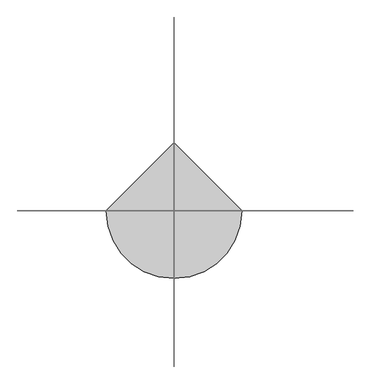
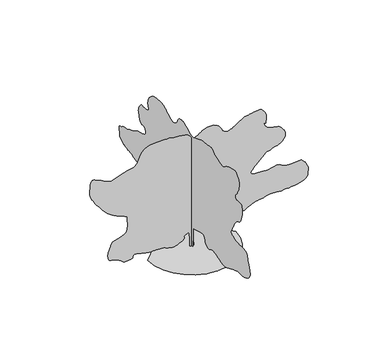
"""IFC4 building model written with IfcOpenShell, lengths in millimetres: geographic element geometry, RPC 木 - 落葉樹 : ヤマボウシ - 3.0 メートル."""

from ifc_helpers import new_model, si_unit, origin, place, context, project, spatial, triangles, source, transform, mapped, element, save


def geographic_element_e0625334(model_context):
    return source(origin(), model_context, "Body", "Tessellation", [
        triangles([(0.0321152, 48.5607305, 0.0034119), (0.0321152, -50.059231, 0.0034119), (0.0321152, -56.2224767, 326.6823853), (0.0321152, -56.2224767, 468.4473149), (0.0321152, -179.4974194, 505.4297959), (0.0321152, -382.8998477, 573.2297636), (0.0321152, -481.5198092, 585.5572815), (0.0321152, -493.3798047, 574.9372539), (0.0321152, -505.079781, 563.9947895), (0.0321152, -516.4547771, 552.4022922), (0.0321152, -527.3447737, 539.8422667), (0.0321152, -537.5872808, 525.9872984), (0.0321152, -547.022279, 510.5148053), (0.0321152, -555.4847712, 493.1023144), (0.0321152, -561.4697619, 475.007307), (0.0321152, -564.8647582, 457.7723125), (0.0321152, -567.614772, 441.509824), (0.0321152, -571.6572578, 426.3248134), (0.0321152, -578.9372641, 412.3273393), (0.0321152, -591.3897743, 399.6223372), (0.0321152, -610.9597281, 388.3173586), (0.0321152, -633.9972754, 377.894848), (0.0321152, -655.6322193, 368.3348574), (0.0321152, -675.9747276, 360.4998705), (0.0321152, -695.1297358, 355.2548418), (0.0321152, -713.2071934, 353.4573498), (0.0321152, -730.3171955, 355.9723489), (0.0321152, -746.5597361, 363.6648663), (0.0321152, -762.949724, 373.6898357), (0.0321152, -780.3097109, 382.7473497), (0.0321152, -798.4772066, 390.9973549), (0.0321152, -817.2921919, 398.597327), (0.0321152, -836.5896332, 405.7148432), (0.0321152, -856.2146708, 412.5073428), (0.0321152, -875.999655, 419.137316), (0.0321152, -993.1095852, 400.6448401), (0.0321152, -1024.8096125, 390.0973372), (0.0321152, -1056.5095671, 379.6573494), (0.0321152, -1088.2070509, 369.4323558), (0.0321152, -1119.9070782, 359.5298716), (0.0321152, -1151.6070328, 350.0598464), (0.0321152, -1183.3045166, 341.1298682), (0.0321152, -1215.0045439, 332.8448725), (0.0321152, -1247.7819763, 324.7573574), (0.0321152, -1282.4994793, 317.2098893), (0.0321152, -1318.8344707, 311.4973746), (0.0321152, -1356.4644413, 308.9098872), (0.0321152, -1395.0644108, 310.7423698), (0.0321152, -1434.3118698, 318.2898743), (0.0321152, -1473.8818382, 332.8448725), (0.0321152, -1769.7418316, 456.1198334), (0.0321152, -1791.6092468, 465.9673064), (0.0321152, -1811.1067486, 474.5198004), (0.0321152, -1830.3892925, 481.9973236), (0.0321152, -1851.611689, 488.6098197), (0.0321152, -1876.9318005, 494.5747899), (0.0321152, -1908.5067627, 500.1098082), (0.0321152, -1948.4892059, 505.4297959), (0.0321152, -1993.2716469, 509.077284), (0.0321152, -2037.2967213, 510.4597941), (0.0321152, -2079.8141842, 511.0898066), (0.0321152, -2120.0666691, 512.4747874), (0.0321152, -2157.3016056, 516.1222755), (0.0321152, -2190.7616272, 523.5422805), (0.0321152, -2219.6915474, 536.2472826), (0.0321152, -2247.0266521, 550.8047879), (0.0321152, -2275.3291397, 563.6347824), (0.0321152, -2303.3066471, 576.0347523), (0.0321152, -2329.6691368, 589.2947714), (0.0321152, -2353.1216297, 604.7147604), (0.0321152, -2372.3665306, 623.5822861), (0.0321152, -2386.1140926, 647.1947256), (0.0321152, -2397.2190834, 669.6572353), (0.0321152, -2408.5415028, 686.5147093), (0.0321152, -2418.7840462, 701.2122133), (0.0321152, -2426.65406, 717.2072399), (0.0321152, -2430.8590359, 737.9447096), (0.0321152, -2430.1039948, 766.8771732), (0.0321152, -2423.0965736, 807.4521675), (0.0321152, -2412.5114639, 849.5371714), (0.0321152, -2401.8190933, 882.9996637), (0.0321152, -2390.9114742, 911.2846378), (0.0321152, -2379.6814911, 937.8421011), (0.0321152, -2368.0191216, 966.1271479), (0.0321152, -2355.8165234, 999.5895676), (0.0321152, -2342.9690517, 1041.6745714), (0.0321152, -2331.7716248, 1086.8520464), (0.0321152, -2322.0866055, 1126.8520758), (0.0321152, -2310.1366081, 1161.0320389), (0.0321152, -2292.1490433, 1188.7420481), (0.0321152, -2264.3491413, 1209.3345411), (0.0321152, -2222.9641674, 1222.1644993), (0.0321152, -2164.2192066, 1226.5870491), (0.0321152, -2098.4666794, 1226.6770145), (0.0321152, -2038.2142525, 1227.3044472), (0.0321152, -1982.9192265, 1229.0120464), (0.0321152, -1932.0467503, 1232.3369888), (0.0321152, -1885.0542698, 1237.8170322), (0.0321152, -1841.4043179, 1245.9944401), (0.0321152, -1800.5592819, 1257.4044994), (0.0321152, -1760.9542866, 1269.0494282), (0.0321152, -1722.9643089, 1278.862056), (0.0321152, -1688.9643494, 1288.7794739), (0.0321152, -1661.3267921, 1300.7495281), (0.0321152, -1642.4218414, 1316.7069843), (0.0321152, -1634.6243523, 1338.5944565), (0.0321152, -1640.3019127, 1368.3519424), (0.0321152, -1650.8868771, 1395.324424), (0.0321152, -1657.8043327, 1411.2994663), (0.0321152, -1663.4292801, 1421.8844307), (0.0321152, -1670.131778, 1432.6844982), (0.0321152, -1680.2843559, 1449.3068848), (0.0321152, -1696.261869, 1477.3593876), (0.0321152, -1720.43176, 1522.4468971), (0.0321152, -1744.7792564, 1570.2993542), (0.0321152, -1762.0142509, 1605.6469059), (0.0321152, -1775.5817368, 1632.5843605), (0.0321152, -1788.931794, 1655.2092876), (0.0321152, -1805.5192989, 1677.6167862), (0.0321152, -1828.7892448, 1703.9067513), (0.0321152, -1862.1967987, 1738.1767525), (0.0321152, -1899.9867886, 1769.4617615), (0.0321152, -1934.3291691, 1788.456823), (0.0321152, -1965.5416534, 1801.7368263), (0.0321152, -1993.9516926, 1815.879277), (0.0321152, -2019.8841213, 1837.4618259), (0.0321152, -2043.6591236, 1873.0592171), (0.0321152, -2065.5992088, 1929.2517174), (0.0321152, -2083.3542297, 1999.8741508), (0.0321152, -2094.4241936, 2071.5741348), (0.0321152, -2098.9166519, 2140.1491642), (0.0321152, -2096.9391563, 2201.391647), (0.0321152, -2088.6017292, 2251.0966072), (0.0321152, -2074.0091606, 2285.0590691), (0.0321152, -2053.2716183, 2299.0765274), (0.0321152, -2028.7792179, 2300.9990845), (0.0321152, -2002.9916931, 2301.6291332), (0.0321152, -1976.1267632, 2301.1790154), (0.0321152, -1948.3992405, 2299.8665955), (0.0321152, -1920.0242283, 2297.9090115), (0.0321152, -1891.2193005, 2295.5190411), (0.0321152, -1862.1967987, 2292.9116421), (0.0321152, -1846.526825, 2300.944146), (0.0321152, -1831.9342564, 2309.6241394), (0.0321152, -1819.4992596, 2319.5991119), (0.0321152, -1810.2992397, 2331.5116116), (0.0321152, -1805.4117474, 2346.0140694), (0.0321152, -1805.914333, 2363.7490334), (0.0321152, -1812.8867271, 2385.36908), (0.0321152, -1823.1842091, 2405.136478), (0.0321152, -1833.371814, 2418.9715347), (0.0321152, -1844.1018276, 2430.0064716), (0.0321152, -1856.0143272, 2441.3640633), (0.0321152, -1869.7617439, 2456.1715897), (0.0321152, -1885.9892418, 2477.5540054), (0.0321152, -1905.3416943, 2508.6489098), (0.0321152, -1927.1592579, 2549.7490173), (0.0321152, -1948.5442898, 2597.4240143), (0.0321152, -1966.7992802, 2649.1990517), (0.0321152, -1979.2367477, 2702.5739914), (0.0321152, -1983.1542412, 2755.098983), (0.0321152, -1975.8567215, 2804.2988869), (0.0321152, -1954.6517658, 2847.6488571), (0.0321152, -1927.4992081, 2886.8737885), (0.0321152, -1902.7191799, 2923.7238647), (0.0321152, -1878.1542549, 2955.8489388), (0.0321152, -1851.6491867, 2980.8488663), (0.0321152, -1821.0442234, 2996.3487923), (0.0321152, -1784.1893509, 2999.9988602), (0.0321152, -1738.9217651, 2989.4239243), (0.0321152, -1692.8293751, 2973.9487061), (0.0321152, -1653.2043228, 2962.998793), (0.0321152, -1617.4618824, 2954.3237411), (0.0321152, -1583.0144211, 2945.6486893), (0.0321152, -1547.2718353, 2934.6987762), (0.0321152, -1507.6469284, 2919.2238487), (0.0321152, -1461.554393, 2896.9487549), (0.0321152, -1417.7968895, 2870.823896), (0.0321152, -1383.95942, 2846.4239319), (0.0321152, -1355.6194347, 2825.4737572), (0.0321152, -1328.3594707, 2809.698848), (0.0321152, -1297.7569782, 2800.8238083), (0.0321152, -1259.3920235, 2800.5738235), (0.0321152, -1208.841984, 2810.6737885), (0.0321152, -1151.1220333, 2827.7739075), (0.0321152, -1095.7745396, 2846.3989334), (0.0321152, -1045.1695616, 2864.9989609), (0.0321152, -1001.6820997, 2882.1237877), (0.0321152, -967.6821402, 2896.1988007), (0.0321152, -945.5421398, 2905.7737976), (0.0321152, -937.6370991, 2909.2738747), (0.0321152, -933.2696331, 2914.6738358), (0.0321152, -920.8171228, 2928.2738777), (0.0321152, -901.2471691, 2946.1489494), (0.0321152, -875.532169, 2964.4987015), (0.0321152, -844.642194, 2979.3736656), (0.0321152, -809.5471704, 2986.9237862), (0.0321152, -771.2146992, 2983.2487198), (0.0321152, -721.277195, 2972.4237991), (0.0321152, -656.2422112, 2961.4738861), (0.0321152, -584.4172711, 2951.0739395), (0.0321152, -514.0997972, 2941.8489212), (0.0321152, -453.5948058, 2934.47379), (0.0321152, -411.2023353, 2929.5487999), (0.0321152, -395.2273293, 2927.7739082), (0.0321152, -389.2073479, 2924.6238098), (0.0321152, -372.7298653, 2916.1987427), (0.0321152, -348.1648676, 2903.9989059), (0.0321152, -317.8848845, 2889.5489159), (0.0321152, -284.2623909, 2874.3239731), (0.0321152, -249.6706434, 2859.8489845), (0.0321152, -216.4799186, 2847.6488571), (0.0321152, -182.6961704, 2835.2237434), (0.0321152, -145.4621876, 2820.7737534), (0.0321152, -105.8562113, 2806.7237389), (0.0321152, -64.9562232, 2795.5988365), (0.0321152, -23.8407913, 2789.8738953), (0.0321152, 16.4121432, 2792.023764), (0.0321152, 54.724226, 2804.4988747), (0.0321152, 95.0672077, 2825.5987495), (0.0321152, 140.4776899, 2850.2489891), (0.0321152, 188.4756686, 2875.9988708), (0.0321152, 236.5816531, 2900.3238396), (0.0321152, 282.3148899, 2920.7737541), (0.0321152, 323.1973872, 2934.8487671), (0.0321152, 356.7473742, 2940.0987373), (0.0321152, 387.7448281, 2939.8987495), (0.0321152, 421.3323492, 2938.5238335), (0.0321152, 455.5648164, 2934.7737717), (0.0321152, 488.5048116, 2927.4489281), (0.0321152, 518.2072864, 2915.3987915), (0.0321152, 542.7372934, 2897.3987274), (0.0321152, 560.1497844, 2872.298806), (0.0321152, 571.7222611, 2845.0237267), (0.0321152, 581.032267, 2820.8737473), (0.0321152, 589.584761, 2799.1989075), (0.0321152, 598.8947668, 2779.3739548), (0.0321152, 610.4672436, 2760.6989319), (0.0321152, 625.8122372, 2742.5988739), (0.0321152, 646.4422279, 2724.3738235), (0.0321152, 671.2597538, 2707.0990059), (0.0321152, 697.802247, 2692.6490158), (0.0321152, 725.529697, 2681.5238228), (0.0321152, 753.9047092, 2674.2739746), (0.0321152, 782.3872004, 2671.4488564), (0.0321152, 810.4371597, 2673.5990158), (0.0321152, 837.5196636, 2681.2238411), (0.0321152, 865.1921751, 2693.0489914), (0.0321152, 895.1296646, 2707.1490028), (0.0321152, 926.9546116, 2723.1238998), (0.0321152, 960.2896408, 2740.598996), (0.0321152, 994.7570864, 2759.2240219), (0.0321152, 1029.9771023, 2778.5990021), (0.0321152, 1065.5771095, 2798.3489594), (0.0321152, 1088.2370636, 2814.0738716), (0.0321152, 1112.1370583, 2829.173822), (0.0321152, 1138.5170614, 2842.9738518), (0.0321152, 1168.617041, 2854.848999), (0.0321152, 1203.6770376, 2864.0987251), (0.0321152, 1244.9369465, 2870.1489372), (0.0321152, 1293.6344101, 2872.298806), (0.0321152, 1349.6844772, 2871.0988792), (0.0321152, 1409.9369041, 2867.1988266), (0.0321152, 1471.0519238, 2860.1739647), (0.0321152, 1529.689333, 2849.5987381), (0.0321152, 1582.5044231, 2835.0237556), (0.0321152, 1626.1519043, 2816.0237526), (0.0321152, 1657.2943348, 2792.1737549), (0.0321152, 1679.9917866, 2768.8240173), (0.0321152, 1700.7467697, 2750.1989914), (0.0321152, 1719.8842644, 2734.2738007), (0.0321152, 1737.7292507, 2718.9988609), (0.0321152, 1754.6017673, 2702.3240067), (0.0321152, 1770.8292652, 2682.1990723), (0.0321152, 1786.7342537, 2656.5738922), (0.0321152, 1800.3918503, 2627.8738998), (0.0321152, 1809.9517319, 2599.8238678), (0.0321152, 1815.8442501, 2572.2990944), (0.0321152, 1818.5042622, 2545.2240028), (0.0321152, 1818.361829, 2518.4738914), (0.0321152, 1815.8442501, 2491.9316162), (0.0321152, 1811.3892895, 2465.4966019), (0.0321152, 1804.2368191, 2441.5614349), (0.0321152, 1794.9292477, 2421.93647), (0.0321152, 1785.8343086, 2405.6565044), (0.0321152, 1779.3293278, 2391.7465977), (0.0321152, 1777.7842186, 2379.241547), (0.0321152, 1783.5718014, 2367.1640865), (0.0321152, 1799.0618443, 2354.5490135), (0.0321152, 1819.8892067, 2343.1016018), (0.0321152, 1840.3917343, 2334.6740639), (0.0321152, 1861.0042843, 2328.511504), (0.0321152, 1882.1543015, 2323.8565556), (0.0321152, 1904.2767883, 2319.9565029), (0.0321152, 1927.7991898, 2316.0565956), (0.0321152, 1953.1541828, 2311.404118), (0.0321152, 1979.1941631, 2310.0565258), (0.0321152, 2004.4766315, 2314.2065632), (0.0321152, 2029.006675, 2320.2990692), (0.0321152, 2052.7816772, 2324.7740868), (0.0321152, 2075.7991676, 2324.0715134), (0.0321152, 2098.064233, 2314.6390949), (0.0321152, 2119.5741119, 2292.9116421), (0.0321152, 2140.2241596, 2265.2015602), (0.0321152, 2159.4692059, 2239.5416439), (0.0321152, 2176.6665573, 2214.9591328), (0.0321152, 2191.1691605, 2190.4841732), (0.0321152, 2202.326619, 2165.1441502), (0.0321152, 2209.4966755, 2137.9741516), (0.0321152, 2212.0315498, 2107.9990917), (0.0321152, 2208.9766491, 2074.5041885), (0.0321152, 2200.421648, 2037.7741631), (0.0321152, 2187.286694, 1998.3467731), (0.0321152, 2170.4840858, 1956.7642822), (0.0321152, 2150.9316456, 1913.5643028), (0.0321152, 2129.5490845, 1869.2867729), (0.0321152, 2107.2466667, 1824.469305), (0.0321152, 2067.8742153, 1829.4092651), (0.0321152, 2030.0117008, 1832.3042919), (0.0321152, 1995.1692055, 1831.0992783), (0.0321152, 1964.8517246, 1823.7492908), (0.0321152, 1940.5742821, 1808.2067802), (0.0321152, 1923.8441986, 1782.4192554), (0.0321152, 1916.1717018, 1744.3393124), (0.0321152, 1917.9141827, 1705.0943241), (0.0321152, 1927.8516575, 1675.6593475), (0.0321152, 1945.1216789, 1653.7718754), (0.0321152, 1968.8591835, 1637.1667843), (0.0321152, 1998.2041946, 1623.5818577), (0.0321152, 2032.2941196, 1610.7493561), (0.0321152, 2070.2641857, 1596.4093884), (0.0321152, 2106.9241573, 1584.1719086), (0.0321152, 2139.3791531, 1577.001852), (0.0321152, 2170.2141895, 1571.6668579), (0.0321152, 2202.0215504, 1564.9268623), (0.0321152, 2237.3865429, 1553.5518299), (0.0321152, 2278.8966545, 1534.306929), (0.0321152, 2329.1415527, 1503.9544212), (0.0321152, 2383.0889866, 1471.1769161), (0.0321152, 2433.9089951, 1445.5168545), (0.0321152, 2481.4915558, 1425.0294422), (0.0321152, 2525.7240303, 1407.7794777), (0.0321152, 2566.5238655, 1391.8218761), (0.0321152, 2603.7489189, 1375.2169304), (0.0321152, 2637.3239044, 1356.0244972), (0.0321152, 2670.0739403, 1339.9419033), (0.0321152, 2704.5488708, 1331.5145107), (0.0321152, 2740.1990204, 1327.0745201), (0.0321152, 2776.4988396, 1322.9595097), (0.0321152, 2812.8989433, 1315.5019707), (0.0321152, 2848.8737823, 1301.0370106), (0.0321152, 2883.8739716, 1275.8969753), (0.0321152, 2917.2239708, 1253.1644966), (0.0321152, 2947.6738564, 1243.4770065), (0.0321152, 2973.7987152, 1239.5070454), (0.0321152, 2994.223922, 1233.9169796), (0.0321152, 3007.5236916, 1219.3794949), (0.0321152, 3012.2986908, 1188.5620445), (0.0321152, 3007.1487144, 1134.1295385), (0.0321152, 3000.7738129, 1075.6195925), (0.0321152, 2999.8988663, 1034.3596109), (0.0321152, 3000.198848, 1005.7171005), (0.0321152, 2997.3737297, 985.049612), (0.0321152, 2987.123774, 967.7271229), (0.0321152, 2965.0989555, 949.1096546), (0.0321152, 2927.023954, 924.5646412), (0.0321152, 2887.2487656, 900.7171143), (0.0321152, 2859.3237259, 885.497113), (0.0321152, 2837.74888, 876.2071278), (0.0321152, 2817.0489807, 870.1496487), (0.0321152, 2791.6987839, 864.6321802), (0.0321152, 2756.2489128, 856.9596834), (0.0321152, 2705.1238358, 844.4346485), (0.0321152, 2648.9490669, 832.3046476), (0.0321152, 2600.4988266, 825.8897049), (0.0321152, 2557.7991074, 822.6021875), (0.0321152, 2518.7488747, 819.8521374), (0.0321152, 2481.3116249, 815.0546831), (0.0321152, 2443.4491104, 805.6196486), (0.0321152, 2403.1065147, 788.9621624), (0.0321152, 2353.7965885, 769.6621777), (0.0321152, 2293.9216095, 753.8122004), (0.0321152, 2228.7616333, 741.0897211), (0.0321152, 2163.6016571, 731.1696871), (0.0321152, 2103.7266781, 723.7297342), (0.0321152, 2054.4166065, 718.4472078), (0.0321152, 2020.9567303, 714.9972004), (0.0321152, 1997.8292175, 712.9122259), (0.0321152, 1975.5641521, 711.1496881), (0.0321152, 1953.5141899, 708.5272465), (0.0321152, 1931.0341667, 703.8547119), (0.0321152, 1907.4742676, 695.9472004), (0.0321152, 1882.1917992, 683.6197552), (0.0321152, 1854.5343304, 665.6872015), (0.0321152, 1828.8017441, 646.4947683), (0.0321152, 1807.9217686, 629.8897499), (0.0321152, 1789.194278, 613.932221), (0.0321152, 1769.9317909, 596.6822565), (0.0321152, 1747.4318562, 576.1947716), (0.0321152, 1719.0043762, 550.5347826), (0.0321152, 1681.9493706, 517.7572775), (0.0321152, 1650.1068375, 485.9673211), (0.0321152, 1634.0068027, 462.6973025), (0.0321152, 1625.991885, 445.139835), (0.0321152, 1618.4068829, 430.494835), (0.0321152, 1603.6018272, 415.9573503), (0.0321152, 1573.9143951, 398.7223557), (0.0321152, 1521.691856, 375.9923478), (0.0321152, 1461.9594555, 353.7623457), (0.0321152, 1412.9019848, 338.5423808), (0.0321152, 1371.6069763, 328.2798532), (0.0321152, 1335.1644333, 320.9298657), (0.0321152, 1300.6620335, 314.4448691), (0.0321152, 1265.1894894, 306.7698652), (0.0321152, 1225.8344788, 295.8623733), (0.0321152, 1191.2045431, 285.4223855), (0.0321152, 1167.682069, 279.5098831), (0.0321152, 1149.0120604, 276.6173816), (0.0321152, 1128.939521, 275.2323825), (0.0321152, 1101.212071, 273.8498906), (0.0321152, 1059.5745689, 270.9573891), (0.0321152, 997.7746347, 265.0448866), (0.0321152, 934.502116, 258.197394), (0.0321152, 888.5896568, 253.2924063), (0.0321152, 853.9971462, 250.0024), (0.0321152, 824.687162, 248.0084084), (0.0321152, 794.6246801, 246.9841431), (0.0321152, 757.7671915, 246.6066589), (0.0321152, 708.0797447, 246.5526469), (0.0321152, 660.1722038, 246.9301493), (0.0321152, 628.2222645, 248.0621478), (0.0321152, 605.5422535, 249.9494054), (0.0321152, 585.4522734, 252.5899056), (0.0321152, 561.2647599, 255.9873908), (0.0321152, 526.2948014, 260.1373919), (0.0321152, 473.8573045, 265.0448866), (0.0321152, 415.5448391, 270.9923979), (0.0321152, 366.6123608, 277.9098899), (0.0321152, 325.8748764, 285.2598773), (0.0321152, 292.1448858, 292.5023858), (0.0321152, 264.237396, 299.0973866), (0.0321152, 240.9663963, 304.5073761), (0.0321152, 221.1454041, 308.189873), (0.0321152, 201.9351668, 312.0898893), (0.0321152, 181.431422, 318.2523766), (0.0321152, 159.8491819, 326.3048647), (0.0321152, 137.4046944, 335.8648553), (0.0321152, 114.3129534, 346.5573712), (0.0321152, 90.7902159, 358.0023485), (0.0321152, 67.0517212, 369.8273535), (0.0321152, 30.0694877, 314.3548674), (45.1947341, 0.000153, 0.0), (-47.2612322, 0.000153, 0.0), (-47.2612322, 0.0001391, 228.0581544), (-65.7527225, 0.0001298, 369.8248464), (-189.0271793, 0.0001344, 302.0223716), (-184.0854206, 0.0001344, 286.1373855), (-181.1921742, 0.0001391, 270.0348982), (-182.3961705, 0.0001391, 253.5048934), (-189.7459218, 0.0001391, 236.3244013), (-205.2901764, 0.0001391, 218.2824067), (-231.0771562, 0.0001391, 199.1621711), (-269.154901, 0.0001437, 178.7481737), (-307.0898675, 0.0001437, 161.1374391), (-333.3798689, 0.0001437, 149.5646898), (-351.4773471, 0.0001437, 142.5206975), (-364.827368, 0.0001437, 138.4951983), (-376.8873513, 0.0001437, 135.9796996), (-391.0998559, 0.0001437, 133.4636922), (-410.9223378, 0.0001437, 129.4384473), (-433.0423176, 0.0001437, 125.9342008), (-452.7923112, 0.0001437, 125.5566984), (-471.5697988, 0.0001437, 127.6594498), (-490.7798181, 0.0001437, 131.5946929), (-511.8222836, 0.0001437, 136.716446), (-536.1022696, 0.0001437, 142.3769472), (-565.0147854, 0.0001437, 147.9294426), (-591.0347815, 0.0001437, 153.8776896), (-608.6472602, 0.0001437, 160.7961808), (-622.2672501, 0.0001437, 168.1461864), (-636.3197353, 0.0001437, 175.3879319), (-655.2247587, 0.0001437, 181.9829327), (-683.4022539, 0.0001437, 187.391923), (-725.2722273, 0.0001437, 191.0756734), (-766.9621971, 0.0001437, 193.3399248), (-795.3921478, 0.0001437, 194.8491713), (-816.1646444, 0.0001437, 195.6044304), (-834.8896643, 0.0001437, 195.6039217), (-857.1721704, 0.0001437, 194.8494256), (-888.6196695, 0.0001437, 193.3399248), (-934.8395954, 0.0001437, 191.0756734), (-986.0895922, 0.0001437, 190.8779202), (-1030.1170647, 0.0001437, 194.7774279), (-1068.7520611, 0.0001391, 201.588422), (-1103.8295712, 0.0001391, 210.1239112), (-1137.1820412, 0.0001391, 219.1989205), (-1170.6420628, 0.0001391, 227.6269126), (-1206.044553, 0.0001391, 234.2219134), (-1242.1820274, 0.0001391, 241.0504028), (-1276.2694817, 0.0001391, 249.6041503), (-1307.7719193, 0.0001391, 257.8348979), (-1336.1469315, 0.0001391, 263.6923892), (-1360.854435, 0.0001391, 265.1298923), (-1381.3594334, 0.0001391, 260.0998941), (-1397.1193726, 0.0001391, 246.5491588), (-1406.1569023, 0.0001391, 228.8306545), (-1409.8044994, 0.0001391, 212.7294208), (-1412.4819523, 0.0001391, 198.3536631), (-1418.6094852, 0.0001437, 185.8104243), (-1432.6093575, 0.0001437, 175.208437), (-1458.8994678, 0.0001437, 166.6544352), (-1501.9019302, 0.0001437, 160.2571876), (-1547.4019146, 0.0001437, 155.854186), (-1580.6118061, 0.0001437, 153.71569), (-1605.086911, 0.0001437, 154.5966864), (-1624.3868958, 0.0001437, 159.2506901), (-1642.069392, 0.0001437, 168.4334327), (-1661.6918861, 0.0001437, 182.8994283), (-1686.8143353, 0.0001391, 203.4031732), (-1714.2017624, 0.0001391, 224.6974039), (-1739.1067829, 0.0001391, 241.6791617), (-1762.8268467, 0.0001391, 255.3198988), (-1786.6567875, 0.0001391, 266.5848907), (-1811.8867882, 0.0001344, 276.4523844), (-1839.8118279, 0.0001344, 285.8848937), (-1871.7267403, 0.0001344, 295.8598844), (-1904.1442383, 0.0001344, 304.2498701), (-1932.574189, 0.0001344, 310.1623907), (-1956.796693, 0.0001344, 316.3998734), (-1976.5992634, 0.0001344, 325.7623833), (-1991.7666515, 0.0001344, 341.0548728), (-2002.0817196, 0.0001298, 365.0798598), (-2007.3292191, 0.0001298, 400.642333), (-2009.4667339, 0.0001252, 439.4223424), (-2010.0966373, 0.0001252, 472.3798147), (-2008.4617081, 0.0001252, 501.2397901), (-2003.8067596, 0.0001205, 527.7272721), (-1995.3792217, 0.0001205, 553.5672647), (-1982.4217278, 0.0001205, 580.4872785), (-1964.1817074, 0.0001159, 610.2097738), (-1949.5917549, 0.0001159, 639.8072405), (-1944.056773, 0.0001113, 665.84475), (-1941.5391941, 0.0001113, 689.2946995), (-1936.0042122, 0.0001113, 711.1297039), (-1921.4142597, 0.0001113, 732.3172188), (-1891.7266823, 0.0001066, 753.8271704), (-1840.9068192, 0.0001066, 776.6297029), (-1777.9392963, 0.0001066, 797.8696856), (-1717.5618771, 0.0001066, 815.9846409), (-1662.3568165, 0.000102, 833.8821676), (-1614.9168343, 0.000102, 854.4771315), (-1577.8268017, 0.000102, 880.6771311), (-1553.6743515, 9.74e-05, 915.3946341), (-1545.0494419, 9.74e-05, 961.542108), (-1543.4319534, 9.27e-05, 1005.7846109), (-1539.6568932, 9.27e-05, 1036.2270842), (-1535.3443657, 8.81e-05, 1057.9345528), (-1532.1093887, 8.81e-05, 1075.9745853), (-1531.5719215, 8.81e-05, 1095.4195467), (-1535.3443657, 8.81e-05, 1121.3320639), (-1545.0494419, 8.34e-05, 1158.7820309), (-1552.0394222, 8.34e-05, 1197.3995138), (-1550.4043476, 7.88e-05, 1225.451944), (-1545.8569508, 7.88e-05, 1245.9544716), (-1544.1143246, 7.88e-05, 1261.9295139), (-1550.8893471, 7.88e-05, 1276.3969448), (-1571.894315, 7.42e-05, 1292.3719872), (-1612.8493732, 7.42e-05, 1312.8745148), (-1663.2192638, 7.42e-05, 1334.9595039), (-1709.3843239, 7.42e-05, 1354.4570057), (-1752.4218132, 6.95e-05, 1372.5544476), (-1793.4117531, 6.95e-05, 1390.4344608), (-1833.431694, 6.95e-05, 1409.284473), (-1873.5591866, 6.95e-05, 1430.2919117), (-1914.8717812, 6.49e-05, 1454.6418789), (-1954.7667297, 6.49e-05, 1480.589423), (-1990.9941696, 6.49e-05, 1506.7543957), (-2025.1742054, 6.03e-05, 1534.8593662), (-2058.9217094, 6.03e-05, 1566.6293747), (-2093.8541702, 5.56e-05, 1603.7917866), (-2131.5916924, 5.56e-05, 1648.0717873), (-2173.7491482, 5.1e-05, 1701.1893299), (-2212.079076, 5.1e-05, 1748.4168251), (-2239.6291386, 4.64e-05, 1778.6042267), (-2259.95159, 4.64e-05, 1798.8768265), (-2276.6091488, 4.64e-05, 1816.3417488), (-2293.1590107, 4.17e-05, 1838.1218147), (-2313.1615688, 4.17e-05, 1871.3317062), (-2340.1690773, 3.71e-05, 1923.0842159), (-2369.5866131, 3.71e-05, 1974.4617485), (-2394.369112, 3.25e-05, 2008.0467625), (-2414.404081, 3.25e-05, 2033.2241501), (-2429.5890553, 3.25e-05, 2059.3692112), (-2439.8141579, 2.78e-05, 2095.8666927), (-2444.9714012, 2.32e-05, 2152.0940746), (-2444.9539604, 1.85e-05, 2237.4340691), (-2440.4065636, 1.39e-05, 2329.0465004), (-2431.9790257, 9.3e-06, 2398.9865627), (-2419.5614697, 9.3e-06, 2448.9790054), (-2403.0464893, 4.6e-06, 2480.7488686), (-2382.3290039, 4.6e-06, 2496.024099), (-2357.2965202, 4.6e-06, 2496.5263939), (-2327.8441029, 4.6e-06, 2483.9841362), (-2296.1790298, 4.6e-06, 2467.2014397), (-2264.7315308, 4.6e-06, 2453.111602), (-2233.7165634, 9.3e-06, 2440.641433), (-2203.3466148, 9.3e-06, 2428.7090218), (-2173.8391136, 9.3e-06, 2416.2365273), (-2145.4116337, 9.3e-06, 2402.149015), (-2118.2766621, 9.3e-06, 2385.3639931), (-2092.0391647, 1.39e-05, 2368.6715527), (-2066.1266476, 1.39e-05, 2355.2116184), (-2040.4841721, 1.39e-05, 2344.4465778), (-2015.0566544, 1.39e-05, 2335.839109), (-1989.789156, 1.39e-05, 2328.8491287), (-1964.6316799, 1.39e-05, 2322.9365536), (-1939.5292877, 1.39e-05, 2317.5640617), (-1655.9942688, 9.3e-06, 2416.1840595), (-1606.9367981, 9.3e-06, 2430.3440964), (-1556.3693905, 9.3e-06, 2441.9166458), (-1506.5568787, 4.6e-06, 2452.0863739), (-1459.7619152, 4.6e-06, 2462.0439056), (-1418.2519489, 4.6e-06, 2472.9691109), (-1384.2894871, 4.6e-06, 2486.0514519), (-1360.1368916, 4.6e-06, 2502.473996), (-1342.0595066, 4.6e-06, 2521.7239838), (-1324.9519753, 0.0, 2542.47388), (-1309.029546, 0.0, 2564.7489738), (-1294.509502, 0.0, 2588.5239761), (-1281.6069466, -4.6e-06, 2613.7988869), (-1270.5394535, -4.6e-06, 2640.5989952), (-1261.5170391, -4.6e-06, 2668.899012), (-1252.17197, -9.3e-06, 2697.4990105), (-1240.346965, -9.3e-06, 2724.7737991), (-1226.5819622, -9.3e-06, 2750.2489883), (-1211.4170448, -1.39e-05, 2773.3490318), (-1195.3869913, -1.39e-05, 2793.5239632), (-1179.0345011, -1.39e-05, 2810.2488144), (-1162.8970413, -1.39e-05, 2822.9989082), (-1145.3595217, -1.39e-05, 2835.8739944), (-1123.7220343, -1.85e-05, 2852.0988762), (-1096.9120428, -1.85e-05, 2869.7239632), (-1063.8470552, -1.85e-05, 2886.8237915), (-1023.4495937, -1.85e-05, 2901.4237724), (-974.6421078, -1.85e-05, 2911.6237312), (-916.3471195, -1.85e-05, 2915.4487885), (-850.4696726, -1.85e-05, 2916.7487091), (-781.7871643, -2.32e-05, 2919.7488167), (-713.5371878, -2.32e-05, 2923.1988968), (-648.9522491, -2.32e-05, 2925.7987381), (-591.2697598, -2.32e-05, 2926.2237122), (-543.7197916, -2.32e-05, 2923.1988968), (-509.5422993, -1.85e-05, 2915.4487885), (-481.004797, -1.85e-05, 2906.6237457), (-448.8023294, -1.85e-05, 2900.6988167), (-413.797344, -1.85e-05, 2896.848761), (-376.8498536, -1.85e-05, 2894.1739243), (-338.824849, -1.85e-05, 2891.823777), (-300.5848866, -1.85e-05, 2888.923954), (-262.9923956, -1.85e-05, 2884.6239258), (-225.8116528, -1.85e-05, 2879.5489449), (-188.9551815, -1.85e-05, 2874.2739761), (-153.5001872, -1.85e-05, 2867.79879), (-120.5252014, -1.85e-05, 2859.173735), (-91.1082107, -1.85e-05, 2847.4238708), (-66.327474, -1.39e-05, 2831.5739662), (-47.2612322, -1.39e-05, 2810.6737885), (-31.5194878, -1.39e-05, 2787.7240265), (-16.4247435, -1.39e-05, 2766.8488472), (-2.6237239, -9.3e-06, 2748.5488014), (9.2364712, -9.3e-06, 2733.3988541), (18.5090174, -9.3e-06, 2721.8989746), (24.5469392, -9.3e-06, 2714.5988388), (26.7032393, -9.3e-06, 2712.0489944), (32.9569863, -9.3e-06, 2714.1738647), (49.5612281, -9.3e-06, 2720.0987938), (73.2819686, -9.3e-06, 2729.0238304), (100.8839584, -9.3e-06, 2740.2240189), (129.1329518, -9.3e-06, 2752.9238251), (154.7941853, -1.39e-05, 2766.3738762), (174.6331814, -1.39e-05, 2779.8489258), (195.6221801, -1.39e-05, 2795.3488518), (224.805664, -1.39e-05, 2814.0988701), (259.0573887, -1.39e-05, 2834.0238167), (295.2473854, -1.85e-05, 2853.0988152), (330.2548779, -1.85e-05, 2869.2489922), (360.9473722, -1.85e-05, 2880.4488899), (384.199841, -1.85e-05, 2884.6239258), (532.1298014, -1.85e-05, 2878.4737198), (558.4372799, -1.85e-05, 2865.2489456), (584.099776, -1.85e-05, 2851.8988884), (608.4672566, -1.39e-05, 2838.3488434), (630.8922323, -1.39e-05, 2824.4738182), (650.7322277, -1.39e-05, 2810.173819), (667.3372461, -1.39e-05, 2795.3238533), (680.0597254, -1.39e-05, 2779.8489258), (690.2672419, -1.39e-05, 2763.8240318), (699.8271961, -9.3e-06, 2747.473867), (708.8472124, -9.3e-06, 2730.8490097), (717.4372404, -9.3e-06, 2713.9988754), (725.7022156, -9.3e-06, 2696.999041), (733.7547037, -4.6e-06, 2679.898922), (741.6971695, -4.6e-06, 2662.7238075), (758.8571686, -4.6e-06, 2650.9239464), (775.9646999, -4.6e-06, 2639.5990562), (792.9646797, -4.6e-06, 2629.2488159), (809.8021694, -4.6e-06, 2620.3490685), (826.4247013, -4.6e-06, 2613.3989113), (842.7771915, -4.6e-06, 2608.8738968), (858.8071724, 0.0, 2607.248996), (876.1296616, -4.6e-06, 2608.7739029), (896.2571394, -4.6e-06, 2613.2989174), (918.9721046, -4.6e-06, 2620.8490379), (944.0571287, -4.6e-06, 2631.3989754), (971.2995792, -4.6e-06, 2644.9990173), (1000.4845711, -4.6e-06, 2661.5988762), (1031.3920595, -4.6e-06, 2681.2238411), (1066.8120632, -9.3e-06, 2705.2988251), (1107.9445816, -9.3e-06, 2733.4738495), (1152.2045254, -1.39e-05, 2763.0487885), (1197.0045525, -1.39e-05, 2791.3488052), (1239.7545593, -1.39e-05, 2815.6487755), (1277.8695293, -1.39e-05, 2833.248864), (1308.7595043, -1.85e-05, 2841.4739433), (1336.0744068, -1.85e-05, 2844.673748), (1365.0069431, -1.85e-05, 2848.8237854), (1395.2869263, -1.85e-05, 2853.773774), (1426.6444599, -1.85e-05, 2859.3737228), (1458.8093571, -1.85e-05, 2865.4739319), (1491.5143375, -1.85e-05, 2871.8738319), (1524.4918304, -1.85e-05, 2878.4737198), (1554.751902, -1.85e-05, 2882.298777), (1584.3143417, -1.85e-05, 2885.2988846), (1612.4719254, -1.85e-05, 2886.7237976), (1638.5293465, -1.85e-05, 2885.6988602), (1661.7818516, -1.85e-05, 2881.4238304), (1681.5318089, -1.85e-05, 2873.1237556), (1697.0743195, -1.85e-05, 2859.9739769), (1712.241853, -1.85e-05, 2841.9739128), (1730.1042801, -1.39e-05, 2820.0737961), (1748.8292999, -1.39e-05, 2794.9488762), (1766.5843208, -1.39e-05, 2767.2488228), (1781.5342804, -9.3e-06, 2737.5988884), (1791.8493484, -9.3e-06, 2706.6490334), (1795.6943172, -4.6e-06, 2675.0489273), (1795.1568501, -4.6e-06, 2644.7990295), (1793.6467678, -4.6e-06, 2617.1239746), (1791.3268513, 0.0, 2591.5990791), (1788.3617706, 0.0, 2567.8240768), (1784.9118359, 0.0, 2545.3239967), (1781.1392464, 4.6e-06, 2523.6738647), (1777.2043121, 4.6e-06, 2502.473996), (1764.1943504, 4.6e-06, 2507.4989799), (1752.3693455, 4.6e-06, 2511.0240555), (1742.9168701, 4.6e-06, 2511.524025), (1737.0217358, 4.6e-06, 2507.4989799), (1735.871806, 4.6e-06, 2497.4440704), (1740.6517467, 4.6e-06, 2479.8340988), (1752.5492764, 4.6e-06, 2453.1665405), (1769.3142414, 9.3e-06, 2424.4140804), (1787.0518215, 9.3e-06, 2401.2689816), (1804.4642761, 9.3e-06, 2383.2990028), (1820.2592422, 1.39e-05, 2370.0716125), (1833.1442116, 1.39e-05, 2361.1590752), (1841.824205, 1.39e-05, 2356.1265335), (1845.0042435, 1.39e-05, 2354.5465427), (1974.4441624, 1.39e-05, 2323.7266216), (2073.0641602, 1.39e-05, 2305.2366165), (2122.3740864, 1.85e-05, 2280.5815807), (2149.9216782, 1.85e-05, 2248.9715916), (2176.3366356, 2.32e-05, 2217.9015404), (2200.4890858, 2.32e-05, 2187.909185), (2221.2440689, 2.32e-05, 2159.5341728), (2237.4715668, 2.78e-05, 2133.3165871), (2248.0366196, 2.78e-05, 2109.7941856), (2251.8115345, 2.78e-05, 2089.5066158), (2251.524052, 2.78e-05, 2068.1941086), (2249.5115295, 3.25e-05, 2042.0291359), (2244.0490723, 3.25e-05, 2012.1991253), (2233.4116402, 3.71e-05, 1979.8891788), (2215.8715771, 3.71e-05, 1946.2842533), (2189.7066044, 3.71e-05, 1912.5717762), (2153.1916821, 4.17e-05, 1879.9393204), (2114.681678, 4.17e-05, 1854.7792282), (2082.1016899, 4.17e-05, 1840.1892757), (2053.0791882, 4.17e-05, 1832.3893158), (2025.2442593, 4.64e-05, 1827.6092297), (1996.2217575, 4.64e-05, 1822.0742477), (1963.6442402, 4.64e-05, 1812.0117805), (1925.1342361, 4.64e-05, 1793.6467678), (1889.0317886, 4.64e-05, 1776.5918495), (1862.7418236, 4.64e-05, 1769.6742485), (1842.4892807, 4.64e-05, 1767.9317677), (1824.5017159, 4.64e-05, 1766.4042446), (1805.0042141, 4.64e-05, 1760.1318077), (1780.2218605, 5.1e-05, 1744.1567654), (1746.3842457, 5.1e-05, 1713.5167751), (1481.3444641, 6.49e-05, 1460.8044388), (1461.8818439, 6.95e-05, 1433.2019085), (1444.5244732, 6.95e-05, 1406.4095032), (1431.3694622, 6.95e-05, 1381.234441), (1424.5243858, 7.42e-05, 1358.4819054), (1426.0869358, 7.42e-05, 1338.9669628), (1438.1619255, 7.42e-05, 1323.4945061), (1462.854459, 7.42e-05, 1312.8745148), (1495.0193562, 7.42e-05, 1306.9819965), (1528.4793777, 7.42e-05, 1304.2144329), (1563.7743164, 7.42e-05, 1303.1719093), (1601.4393139, 7.42e-05, 1302.4520405), (1642.0143082, 7.42e-05, 1300.6544758), (1686.0418533, 7.42e-05, 1296.379446), (1734.0568005, 7.42e-05, 1288.219479), (1788.6517239, 7.42e-05, 1285.9745579), (1850.0367851, 7.42e-05, 1295.9120327), (1915.1967613, 7.42e-05, 1311.3469917), (1981.1091625, 7.42e-05, 1325.596994), (2044.7592018, 7.42e-05, 1331.9769825), (2103.1267147, 7.42e-05, 1323.8019001), (2153.1916821, 7.42e-05, 1294.3845097), (2211.5940765, 7.88e-05, 1263.4945347), (2290.5915802, 7.88e-05, 1251.039481), (2380.5840523, 7.88e-05, 1250.5544815), (2471.979055, 7.88e-05, 1255.569437), (2555.1739769, 7.88e-05, 1259.6120682), (2620.5990532, 7.88e-05, 1256.2144558), (2658.6240578, 7.88e-05, 1238.9095528), (2678.2990196, 7.88e-05, 1215.9270166), (2695.2738556, 8.34e-05, 1198.4420374), (2709.8738365, 8.34e-05, 1184.4069929), (2722.448941, 8.34e-05, 1171.7745518), (2733.2738617, 8.34e-05, 1158.4945484), (2742.7238663, 8.34e-05, 1142.5195787), (2751.073938, 8.81e-05, 1121.7995499), (2759.9239792, 8.81e-05, 1100.8995901), (2769.8739532, 8.81e-05, 1083.6670664), (2779.6989349, 8.81e-05, 1066.9720825), (2788.223996, 9.27e-05, 1047.6896112), (2794.2989159, 9.27e-05, 1022.6946253), (2796.6737709, 9.27e-05, 988.8570831), (2794.2239204, 9.74e-05, 943.0521029), (2791.0988205, 0.000102, 894.8196545), (2788.9739502, 0.000102, 854.5671696), (2782.7487488, 0.000102, 820.4596584), (2767.3238182, 0.0001066, 790.6646748), (2737.6988823, 0.0001066, 763.3496996), (2688.7739616, 0.0001113, 736.682214), (2615.4740753, 0.0001113, 708.8296989), (2533.8991127, 0.0001113, 685.0372559), (2461.6840439, 0.0001113, 670.1947025), (2396.1640606, 0.0001159, 661.9272566), (2334.6365662, 0.0001159, 657.8672573), (2274.3991093, 0.0001159, 655.6372335), (2212.7615925, 0.0001159, 652.8697426), (2147.0266514, 0.0001159, 647.1922548), (2085.8042255, 0.0001159, 644.2622738), (2036.1167061, 0.0001159, 648.6647667), (1992.8966698, 0.0001159, 656.4097155), (1951.0817802, 0.0001113, 663.5097181), (1905.5992367, 0.0001113, 665.9697424), (1851.3842319, 0.0001159, 659.8072552), (1783.3667267, 0.0001159, 641.0272242), (1715.8542778, 0.0001159, 620.4522446), (1663.6517956, 0.0001159, 609.257252), (1622.4442818, 0.0001159, 603.9922754), (1587.9242958, 0.0001159, 601.207271), (1555.7768394, 0.0001159, 597.4497605), (1521.6869144, 0.0001159, 589.2747508), (1481.3444641, 0.0001205, 573.2272565), (1443.3569572, 0.0001205, 555.5272831), (1416.689399, 0.0001205, 543.3247939), (1397.5668743, 0.0001205, 534.5747829), (1382.2218807, 0.0001205, 527.2247955), (1366.8744164, 0.0001205, 519.2272822), (1347.7545078, 0.0001205, 508.5348026), (1321.0869495, 0.0001252, 493.0998073), (1295.0670261, 0.0001252, 477.717316), (1277.4570545, 0.0001252, 467.4023206), (1263.8344849, 0.0001252, 460.4298174), (1249.7819996, 0.0001252, 455.0748027), (1230.8770489, 0.0001252, 449.6123091), (1202.6995537, 0.0001252, 442.3148257), (1160.8295076, 0.0001252, 431.4623268), (895.7896534, 0.0001298, 382.1523643), (840.1546772, 0.0001298, 368.7823591), (796.3796602, 0.0001298, 359.7248451), (758.9647202, 0.0001298, 354.0098597), (722.4146982, 0.0001344, 350.6673675), (681.2272413, 0.0001344, 348.7273696), (629.9047199, 0.0001344, 347.21736), (562.947288, 0.0001344, 345.1698469), (488.7672956, 0.0001344, 343.2448554), (420.0873307, 0.0001344, 342.6173501), (357.874849, 0.0001344, 343.067359), (303.0998857, 0.0001344, 344.3773444), (256.7373995, 0.0001344, 346.3373629), (219.7556634, 0.0001344, 348.7273696), (193.1239314, 0.0001344, 351.3323705), (172.5304391, 0.0001298, 355.5923575), (152.907182, 0.0001298, 362.7623414), (134.092442, 0.0001298, 372.3573589), (115.924701, 0.0001298, 383.8948451), (98.2422138, 0.0001298, 396.8873297), (80.8829718, 0.0001298, 410.8498495), (63.6857248, 0.0001298, 425.2973325), (39.0307344, 0.0001252, 505.4247817), (26.7032393, 0.0001344, 289.69489), (-1057.7445934, 0.0, 0.0031152), (-1029.7795853, -242.364912, 0.0031152), (-950.1421497, -464.9373184, 0.0031152), (-825.2021742, -661.344734, 0.0031152), (-661.344734, -825.204645, 0.0031152), (-464.9373184, -950.1421497, 0.0031152), (-242.364912, -1029.7795853, 0.0031152), (4.62e-05, -1057.7445934, 0.0031152), (242.3651482, -1029.7795853, 0.0031152), (464.9373184, -950.1421497, 0.0031152), (661.344734, -825.2021742, 0.0031152), (825.204645, -661.344734, 0.0031152), (950.1421497, -464.9373184, 0.0031152), (1029.7795853, -242.364912, 0.0031152), (1057.7445934, 9.27e-05, 0.0031152), (-0.0001387, 1057.7445934, 0.0031152)], [[451, 1, 2], [451, 2, 3], [451, 3, 4], [450, 451, 4], [316, 317, 318], [316, 318, 319], [315, 316, 319], [356, 357, 358], [355, 356, 358], [354, 355, 358], [354, 358, 359], [353, 354, 359], [353, 359, 360], [133, 134, 135], [133, 135, 136], [132, 133, 136], [132, 136, 137], [132, 137, 138], [131, 132, 138], [131, 138, 139], [131, 139, 140], [130, 131, 140], [130, 140, 141], [130, 141, 142], [129, 130, 142], [128, 129, 142], [127, 128, 142], [126, 127, 142], [125, 126, 142], [124, 125, 142], [123, 124, 142], [122, 123, 142], [122, 142, 143], [121, 122, 143], [121, 143, 144], [121, 144, 145], [120, 121, 145], [119, 120, 145], [119, 145, 146], [118, 119, 146], [315, 319, 320], [314, 315, 320], [313, 314, 320], [312, 313, 320], [311, 312, 320], [310, 311, 320], [309, 310, 320], [308, 309, 320], [307, 308, 320], [306, 307, 320], [305, 306, 320], [304, 305, 320], [304, 320, 321], [303, 304, 321], [302, 303, 321], [301, 302, 321], [300, 301, 321], [299, 300, 321], [298, 299, 321], [297, 298, 321], [296, 297, 321], [295, 296, 321], [294, 295, 321], [293, 294, 321], [292, 293, 321], [292, 321, 322], [291, 292, 322], [290, 291, 322], [289, 290, 322], [289, 322, 323], [288, 289, 323], [352, 353, 360], [352, 360, 361], [117, 118, 146], [351, 352, 361], [350, 351, 361], [349, 350, 361], [348, 349, 361], [347, 348, 361], [347, 361, 362], [347, 362, 363], [347, 363, 364], [347, 364, 365], [347, 365, 366], [347, 366, 367], [347, 367, 368], [347, 368, 369], [347, 369, 370], [347, 370, 371], [347, 371, 372], [347, 372, 373], [347, 373, 374], [346, 347, 374], [346, 374, 375], [346, 375, 376], [345, 346, 376], [345, 376, 377], [344, 345, 377], [343, 344, 377], [343, 377, 378], [342, 343, 378], [341, 342, 378], [341, 378, 379], [340, 341, 379], [340, 379, 380], [340, 380, 381], [339, 340, 381], [339, 381, 382], [339, 382, 383], [338, 339, 383], [338, 383, 384], [337, 338, 384], [337, 384, 385], [336, 337, 385], [335, 336, 385], [334, 335, 385], [333, 334, 385], [333, 385, 386], [332, 333, 386], [332, 386, 387], [332, 387, 388], [331, 332, 388], [331, 388, 389], [331, 389, 390], [330, 331, 390], [329, 330, 390], [329, 390, 391], [328, 329, 391], [328, 391, 392], [328, 392, 393], [327, 328, 393], [327, 393, 394], [327, 394, 395], [327, 395, 396], [326, 327, 396], [326, 396, 397], [326, 397, 398], [326, 398, 399], [326, 399, 400], [326, 400, 401], [326, 401, 402], [325, 326, 402], [288, 323, 324], [116, 117, 146], [116, 146, 147], [115, 116, 147], [114, 115, 147], [113, 114, 147], [112, 113, 147], [111, 112, 147], [110, 111, 147], [325, 402, 403], [204, 205, 206], [167, 168, 169], [167, 169, 170], [166, 167, 170], [165, 166, 170], [165, 170, 171], [164, 165, 171], [164, 171, 172], [163, 164, 172], [162, 163, 172], [161, 162, 172], [160, 161, 172], [159, 160, 172], [158, 159, 172], [158, 172, 173], [157, 158, 173], [157, 173, 174], [156, 157, 174], [156, 174, 175], [155, 156, 175], [155, 175, 176], [154, 155, 176], [153, 154, 176], [152, 153, 176], [152, 176, 177], [151, 152, 177], [151, 177, 178], [151, 178, 179], [150, 151, 179], [150, 179, 180], [149, 150, 180], [149, 180, 181], [148, 149, 181], [148, 181, 182], [147, 148, 182], [110, 147, 182], [110, 182, 183], [110, 183, 184], [110, 184, 185], [110, 185, 186], [109, 110, 186], [109, 186, 187], [108, 109, 187], [108, 187, 188], [107, 108, 188], [107, 188, 189], [107, 189, 190], [107, 190, 191], [106, 107, 191], [89, 90, 91], [89, 91, 92], [88, 89, 92], [88, 92, 93], [87, 88, 93], [87, 93, 94], [86, 87, 94], [86, 94, 95], [85, 86, 95], [84, 85, 95], [84, 95, 96], [83, 84, 96], [83, 96, 97], [82, 83, 97], [81, 82, 97], [80, 81, 97], [79, 80, 97], [78, 79, 97], [77, 78, 97], [76, 77, 97], [75, 76, 97], [74, 75, 97], [73, 74, 97], [72, 73, 97], [71, 72, 97], [70, 71, 97], [69, 70, 97], [68, 69, 97], [67, 68, 97], [66, 67, 97], [65, 66, 97], [64, 65, 97], [63, 64, 97], [62, 63, 97], [61, 62, 97], [60, 61, 97], [59, 60, 97], [58, 59, 97], [57, 58, 97], [57, 97, 98], [56, 57, 98], [56, 98, 99], [55, 56, 99], [55, 99, 100], [54, 55, 100], [54, 100, 101], [53, 54, 101], [53, 101, 102], [52, 53, 102], [51, 52, 102], [50, 51, 102], [50, 102, 103], [50, 103, 104], [50, 104, 105], [49, 50, 105], [48, 49, 105], [47, 48, 105], [46, 47, 105], [45, 46, 105], [44, 45, 105], [43, 44, 105], [42, 43, 105], [41, 42, 105], [40, 41, 105], [39, 40, 105], [38, 39, 105], [37, 38, 105], [36, 37, 105], [35, 36, 105], [35, 105, 106], [35, 106, 191], [34, 35, 191], [33, 34, 191], [32, 33, 191], [31, 32, 191], [30, 31, 191], [29, 30, 191], [28, 29, 191], [27, 28, 191], [26, 27, 191], [25, 26, 191], [24, 25, 191], [23, 24, 191], [22, 23, 191], [21, 22, 191], [20, 21, 191], [19, 20, 191], [18, 19, 191], [17, 18, 191], [16, 17, 191], [15, 16, 191], [14, 15, 191], [13, 14, 191], [12, 13, 191], [11, 12, 191], [10, 11, 191], [9, 10, 191], [8, 9, 191], [7, 8, 191], [6, 7, 191], [5, 6, 191], [5, 191, 192], [5, 192, 193], [5, 193, 194], [5, 194, 195], [5, 195, 196], [5, 196, 197], [5, 197, 198], [5, 198, 199], [5, 199, 200], [5, 200, 201], [5, 201, 202], [5, 202, 203], [5, 203, 204], [5, 204, 206], [5, 206, 207], [5, 207, 208], [5, 208, 209], [5, 209, 210], [5, 210, 211], [5, 211, 212], [5, 212, 213], [5, 213, 214], [5, 214, 215], [5, 215, 216], [5, 216, 217], [5, 217, 218], [4, 5, 218], [4, 218, 219], [4, 219, 220], [4, 220, 221], [4, 221, 222], [4, 222, 223], [4, 223, 224], [4, 224, 225], [4, 225, 226], [4, 226, 227], [4, 227, 228], [4, 228, 229], [4, 229, 230], [4, 230, 231], [4, 231, 232], [4, 232, 233], [4, 233, 234], [4, 234, 235], [4, 235, 236], [4, 236, 237], [4, 237, 238], [4, 238, 239], [4, 239, 240], [4, 240, 241], [4, 241, 242], [4, 242, 243], [4, 243, 244], [4, 244, 245], [450, 4, 245], [449, 450, 245], [448, 449, 245], [447, 448, 245], [446, 447, 245], [445, 446, 245], [444, 445, 245], [443, 444, 245], [442, 443, 245], [441, 442, 245], [440, 441, 245], [439, 440, 245], [438, 439, 245], [437, 438, 245], [436, 437, 245], [435, 436, 245], [434, 435, 245], [433, 434, 245], [432, 433, 245], [431, 432, 245], [430, 431, 245], [429, 430, 245], [428, 429, 245], [427, 428, 245], [426, 427, 245], [425, 426, 245], [424, 425, 245], [423, 424, 245], [422, 423, 245], [422, 245, 246], [421, 422, 246], [420, 421, 246], [419, 420, 246], [418, 419, 246], [417, 418, 246], [416, 417, 246], [415, 416, 246], [414, 415, 246], [413, 414, 246], [412, 413, 246], [411, 412, 246], [410, 411, 246], [409, 410, 246], [408, 409, 246], [407, 408, 246], [406, 407, 246], [405, 406, 246], [404, 405, 246], [403, 404, 246], [325, 403, 246], [324, 325, 246], [288, 324, 246], [288, 246, 247], [288, 247, 248], [288, 248, 249], [287, 288, 249], [287, 249, 250], [287, 250, 251], [287, 251, 252], [287, 252, 253], [287, 253, 254], [287, 254, 255], [287, 255, 256], [287, 256, 257], [287, 257, 258], [287, 258, 259], [287, 259, 260], [287, 260, 261], [287, 261, 262], [287, 262, 263], [286, 287, 263], [286, 263, 264], [286, 264, 265], [286, 265, 266], [286, 266, 267], [286, 267, 268], [286, 268, 269], [286, 269, 270], [285, 286, 270], [285, 270, 271], [285, 271, 272], [285, 272, 273], [285, 273, 274], [285, 274, 275], [285, 275, 276], [285, 276, 277], [285, 277, 278], [285, 278, 279], [285, 279, 280], [285, 280, 281], [285, 281, 282], [284, 285, 282], [284, 282, 283], [751, 752, 753], [906, 452, 453], [906, 453, 454], [906, 454, 455], [905, 906, 455], [751, 753, 754], [750, 751, 754], [750, 754, 755], [749, 750, 755], [600, 601, 602], [599, 600, 602], [599, 602, 603], [598, 599, 603], [598, 603, 604], [597, 598, 604], [597, 604, 605], [597, 605, 606], [596, 597, 606], [596, 606, 607], [596, 607, 608], [596, 608, 609], [595, 596, 609], [595, 609, 610], [595, 610, 611], [594, 595, 611], [593, 594, 611], [592, 593, 611], [591, 592, 611], [591, 611, 612], [590, 591, 612], [590, 612, 613], [589, 590, 613], [589, 613, 614], [589, 614, 615], [588, 589, 615], [588, 615, 616], [587, 588, 616], [586, 587, 616], [585, 586, 616], [584, 585, 616], [584, 616, 617], [583, 584, 617], [582, 583, 617], [581, 582, 617], [580, 581, 617], [580, 617, 618], [579, 580, 618], [578, 579, 618], [577, 578, 618], [576, 577, 618], [575, 576, 618], [574, 575, 618], [573, 574, 618], [572, 573, 618], [571, 572, 618], [570, 571, 618], [570, 618, 619], [569, 570, 619], [569, 619, 620], [569, 620, 621], [568, 569, 621], [568, 621, 622], [567, 568, 622], [567, 622, 623], [567, 623, 624], [566, 567, 624], [566, 624, 625], [566, 625, 626], [565, 566, 626], [903, 904, 905], [748, 749, 755], [565, 626, 627], [902, 903, 905], [508, 509, 510], [508, 510, 511], [507, 508, 511], [507, 511, 512], [506, 507, 512], [506, 512, 513], [505, 506, 513], [505, 513, 514], [505, 514, 515], [505, 515, 516], [505, 516, 517], [505, 517, 518], [505, 518, 519], [505, 519, 520], [505, 520, 521], [504, 505, 521], [504, 521, 522], [504, 522, 523], [747, 748, 755], [747, 755, 756], [565, 627, 628], [901, 902, 905], [900, 901, 905], [899, 900, 905], [898, 899, 905], [897, 898, 905], [896, 897, 905], [895, 896, 905], [894, 895, 905], [893, 894, 905], [892, 893, 905], [825, 826, 827], [824, 825, 827], [824, 827, 828], [823, 824, 828], [823, 828, 829], [823, 829, 830], [823, 830, 831], [823, 831, 832], [823, 832, 833], [823, 833, 834], [823, 834, 835], [822, 823, 835], [822, 835, 836], [822, 836, 837], [822, 837, 838], [822, 838, 839], [822, 839, 840], [822, 840, 841], [822, 841, 842], [822, 842, 843], [822, 843, 844], [822, 844, 845], [822, 845, 846], [822, 846, 847], [822, 847, 848], [822, 848, 849], [822, 849, 850], [821, 822, 850], [821, 850, 851], [821, 851, 852], [821, 852, 853], [820, 821, 853], [820, 853, 854], [820, 854, 855], [820, 855, 856], [820, 856, 857], [819, 820, 857], [819, 857, 858], [818, 819, 858], [817, 818, 858], [816, 817, 858], [815, 816, 858], [814, 815, 858], [814, 858, 859], [813, 814, 859], [813, 859, 860], [812, 813, 860], [812, 860, 861], [812, 861, 862], [811, 812, 862], [810, 811, 862], [810, 862, 863], [809, 810, 863], [809, 863, 864], [808, 809, 864], [808, 864, 865], [807, 808, 865], [807, 865, 866], [806, 807, 866], [806, 866, 867], [805, 806, 867], [805, 867, 868], [805, 868, 869], [804, 805, 869], [804, 869, 870], [804, 870, 871], [804, 871, 872], [804, 872, 873], [804, 873, 874], [804, 874, 875], [804, 875, 876], [804, 876, 877], [804, 877, 878], [804, 878, 879], [804, 879, 880], [804, 880, 881], [804, 881, 882], [804, 882, 883], [803, 804, 883], [803, 883, 884], [803, 884, 885], [803, 885, 886], [803, 886, 887], [803, 887, 888], [803, 888, 889], [803, 889, 890], [803, 890, 891], [802, 803, 891], [802, 891, 892], [802, 892, 905], [801, 802, 905], [800, 801, 905], [799, 800, 905], [688, 689, 690], [746, 747, 756], [905, 455, 456], [768, 769, 770], [767, 768, 770], [767, 770, 771], [767, 771, 772], [767, 772, 773], [767, 773, 774], [767, 774, 775], [767, 775, 776], [767, 776, 777], [767, 777, 778], [767, 778, 779], [767, 779, 780], [767, 780, 781], [767, 781, 782], [767, 782, 783], [767, 783, 784], [767, 784, 785], [767, 785, 786], [767, 786, 787], [767, 787, 788], [767, 788, 789], [766, 767, 789], [766, 789, 790], [766, 790, 791], [766, 791, 792], [766, 792, 793], [766, 793, 794], [766, 794, 795], [765, 766, 795], [764, 765, 795], [763, 764, 795], [763, 795, 796], [762, 763, 796], [761, 762, 796], [761, 796, 797], [761, 797, 798], [760, 761, 798], [759, 760, 798], [758, 759, 798], [757, 758, 798], [745, 746, 756], [744, 745, 756], [743, 744, 756], [742, 743, 756], [741, 742, 756], [740, 741, 756], [739, 740, 756], [738, 739, 756], [737, 738, 756], [736, 737, 756], [735, 736, 756], [734, 735, 756], [733, 734, 756], [732, 733, 756], [731, 732, 756], [730, 731, 756], [729, 730, 756], [728, 729, 756], [727, 728, 756], [726, 727, 756], [726, 756, 757], [726, 757, 798], [725, 726, 798], [724, 725, 798], [723, 724, 798], [722, 723, 798], [721, 722, 798], [720, 721, 798], [719, 720, 798], [718, 719, 798], [717, 718, 798], [716, 717, 798], [715, 716, 798], [714, 715, 798], [713, 714, 798], [712, 713, 798], [711, 712, 798], [710, 711, 798], [710, 798, 799], [710, 799, 905], [709, 710, 905], [708, 709, 905], [707, 708, 905], [706, 707, 905], [705, 706, 905], [704, 705, 905], [703, 704, 905], [702, 703, 905], [701, 702, 905], [700, 701, 905], [699, 700, 905], [698, 699, 905], [697, 698, 905], [696, 697, 905], [695, 696, 905], [694, 695, 905], [693, 694, 905], [692, 693, 905], [691, 692, 905], [690, 691, 905], [688, 690, 905], [687, 688, 905], [686, 687, 905], [685, 686, 905], [684, 685, 905], [683, 684, 905], [682, 683, 905], [681, 682, 905], [680, 681, 905], [679, 680, 905], [678, 679, 905], [677, 678, 905], [676, 677, 905], [675, 676, 905], [674, 675, 905], [674, 905, 456], [673, 674, 456], [672, 673, 456], [671, 672, 456], [670, 671, 456], [669, 670, 456], [668, 669, 456], [667, 668, 456], [666, 667, 456], [665, 666, 456], [664, 665, 456], [663, 664, 456], [662, 663, 456], [661, 662, 456], [660, 661, 456], [659, 660, 456], [658, 659, 456], [657, 658, 456], [656, 657, 456], [655, 656, 456], [654, 655, 456], [653, 654, 456], [652, 653, 456], [651, 652, 456], [650, 651, 456], [649, 650, 456], [648, 649, 456], [647, 648, 456], [646, 647, 456], [645, 646, 456], [644, 645, 456], [643, 644, 456], [642, 643, 456], [641, 642, 456], [640, 641, 456], [639, 640, 456], [638, 639, 456], [637, 638, 456], [636, 637, 456], [635, 636, 456], [634, 635, 456], [633, 634, 456], [632, 633, 456], [631, 632, 456], [630, 631, 456], [629, 630, 456], [628, 629, 456], [565, 628, 456], [564, 565, 456], [563, 564, 456], [562, 563, 456], [561, 562, 456], [560, 561, 456], [559, 560, 456], [558, 559, 456], [557, 558, 456], [556, 557, 456], [555, 556, 456], [554, 555, 456], [553, 554, 456], [552, 553, 456], [551, 552, 456], [551, 456, 457], [551, 457, 458], [551, 458, 459], [551, 459, 460], [551, 460, 461], [551, 461, 462], [551, 462, 463], [551, 463, 464], [551, 464, 465], [551, 465, 466], [551, 466, 467], [551, 467, 468], [551, 468, 469], [551, 469, 470], [551, 470, 471], [551, 471, 472], [551, 472, 473], [551, 473, 474], [551, 474, 475], [551, 475, 476], [551, 476, 477], [551, 477, 478], [551, 478, 479], [551, 479, 480], [551, 480, 481], [551, 481, 482], [551, 482, 483], [551, 483, 484], [551, 484, 485], [551, 485, 486], [551, 486, 487], [551, 487, 488], [551, 488, 489], [551, 489, 490], [551, 490, 491], [551, 491, 492], [551, 492, 493], [551, 493, 494], [551, 494, 495], [551, 495, 496], [551, 496, 497], [551, 497, 498], [551, 498, 499], [551, 499, 500], [551, 500, 501], [551, 501, 502], [551, 502, 503], [551, 503, 504], [551, 504, 523], [550, 551, 523], [549, 550, 523], [548, 549, 523], [548, 523, 524], [547, 548, 524], [547, 524, 525], [546, 547, 525], [545, 546, 525], [544, 545, 525], [543, 544, 525], [542, 543, 525], [541, 542, 525], [540, 541, 525], [540, 525, 526], [539, 540, 526], [538, 539, 526], [537, 538, 526], [536, 537, 526], [535, 536, 526], [534, 535, 526], [534, 526, 527], [533, 534, 527], [533, 527, 528], [532, 533, 528], [532, 528, 529], [531, 532, 529], [531, 529, 530], [921, 922, 907], [920, 921, 907], [920, 907, 908], [919, 920, 908], [919, 908, 909], [919, 909, 910], [918, 919, 910], [917, 918, 910], [917, 910, 911], [917, 911, 912], [917, 912, 913], [917, 913, 914], [917, 914, 915], [917, 915, 916]], closed=False),
    ])


if __name__ == "__main__":
    model = new_model("IFC4")
    model_context = context("Model", 3, world=origin())
    ifc_project = project(units=[si_unit("LENGTHUNIT", "METRE", prefix="MILLI")], contexts=[model_context])
    site = spatial("IfcSite", under=ifc_project)
    building = spatial("IfcBuilding", under=site)
    placement = place(None, origin())
    geographic_element_shape = geographic_element_e0625334(model_context)
    element("IfcGeographicElement", 1, ObjectType="RPC 木 - 落葉樹 : ヤマボウシ - 3.0 メートル", at=placement, inside=building, context=model_context, shape_type="MappedRepresentation", body=[
        mapped(geographic_element_shape, transform((0.0, 0.0, 0.0), x_axis=(1.0, 0.0, 0.0), y_axis=(0.0, 1.0, 0.0), z_axis=(0.0, 0.0, 1.0))),
    ])
    save(model, "model.ifc")

# Revit data of these elements
# Type "RPC 木 - 落葉樹 : ヤマボウシ - 3.0 メートル"
#   built-in parameter 1005198 = "{2, 15},{39, RPC-16-G2M3-G0FX-C7PN-N000-ST1L-LVER-AU},{1, 0},{1, 0},{2, 35},{1, 8},{5, Color},{1, 0},{1, 0},{3, 0.8},{3, 0.8},{3, 0.8},{1, 8},{7, BBoxMin},{1, 0},{1, 0},{1, 0},{1, 0},{1, 0},{1, 8},{7, BBoxMax},{1, 0},{1, 0},{1, 0},{1, 0},{1, 0},{2, 11},{9, RPCTypeId},{1, 0},{1, 0},{39, RPC-16-G2M3-G0FX-C7PN-N000-ST1L-LVER-AU},{1, 6},{14, RPCPlantHeight},{1, 0},{1, 0},{7, 9.84252},{2, 11},{7, keyword},{1, 0},{1, 0},{134, :Geometry:RPC:Kousa Dogwood:Cornus kousa:very small trees:native to eastern Asia:occasionally planted in Canada and the United States.},{2, 11},{8, category},{1, 0},{1, 0},{16, :Trees [General]},{2, 11},{12, LocalizedUID},{1, 0},{1, 0},{13, Kousa Dogwood},{2, 14},{6, Height},{1, 0},{1, 0},{7, 9.84252},{1, 2},{16, Cast Reflections},{1, 0},{1, 0},{1, 0},{1, 2},{12, Cast Shadows},{1, 0},{1, 0},{1, 1},{1, 2},{9, Lock View},{1, 0},{1, 0},{1, 0},{1, 4},{5, ViewC},{1, 0},{1, 0},{1, 0},{2, 11},{20, AdvancedUIDefinition},{1, 0},{1, 0},{0, },{2, 11},{10, AssetLibID},{1, 0},{1, 0},{36, 4D3F6E72-3F99-4203-98E9-AF80B3C7A7A4},{2, 11},{10, BaseSchema},{1, 0},{1, 0},{9, RPCSchema},{2, 11},{12, ExchangeGUID},{1, 0},{1, 0},{0, },{1, 2},{6, Hidden},{1, 0},{1, 0},{1, 0},{1, 4},{11, RPCCategory},{1, 0},{1, 0},{1, 0},{2, 11},{8, RPCImage},{1, 0},{1, 0},{0, },{1, 4},{13, SchemaVersion},{1, 0},{1, 0},{1, 4},{2, 11},{12, UIDefinition},{1, 0},{1, 0},{0, },{2, 11},{6, UIName},{1, 0},{1, 0},{39, RPC-16-G2M3-G0FX-C7PN-N000-ST1L-LVER-AU},{2, 11},{11, VersionGUID},{1, 0},{1, 0},{9, RPCSchema},{2, 11},{9, assettype},{1, 0},{1, 0},{11, RPCGeometry},{2, 11},{11, description},{1, 0},{1, 0},{0, },{2, 11},{9, localname},{1, 0},{1, 0},{3, RPC},{2, 11},{9, localtype},{1, 0},{1, 0},{3, RPC},{1, 4},{8, revision},{1, 0},{1, 0},{1, 1},{2, 11},{9, thumbnail},{1, 0},{1, 0},{0, },{1, 4},{7, version},{1, 0},{1, 0},{1, 1},{1, 2},{20, RPC_Cast Reflections},{1, 0},{1, 0},{1, 1},{1, 2},{16, RPC_Cast Shadows},{1, 0},{1, 0},{1, 1},{1, 2},{13, RPC_Lock View},{1, 0},{1, 0},{1, 0},{1, 4},{9, RPC_ViewC},{1, 0},{1, 0},{1, 0},{21, assetlibrary_base.fbx},{1, 5},"
#   built-in parameter 1005195 = "RPC-16-G2M3-G0FX-C7PN-N000-ST1L-LVER-AU"
#   Type Comments = "ヤマボウシ"
#   Height = 3000 mm
#   Default Elevation = 0
